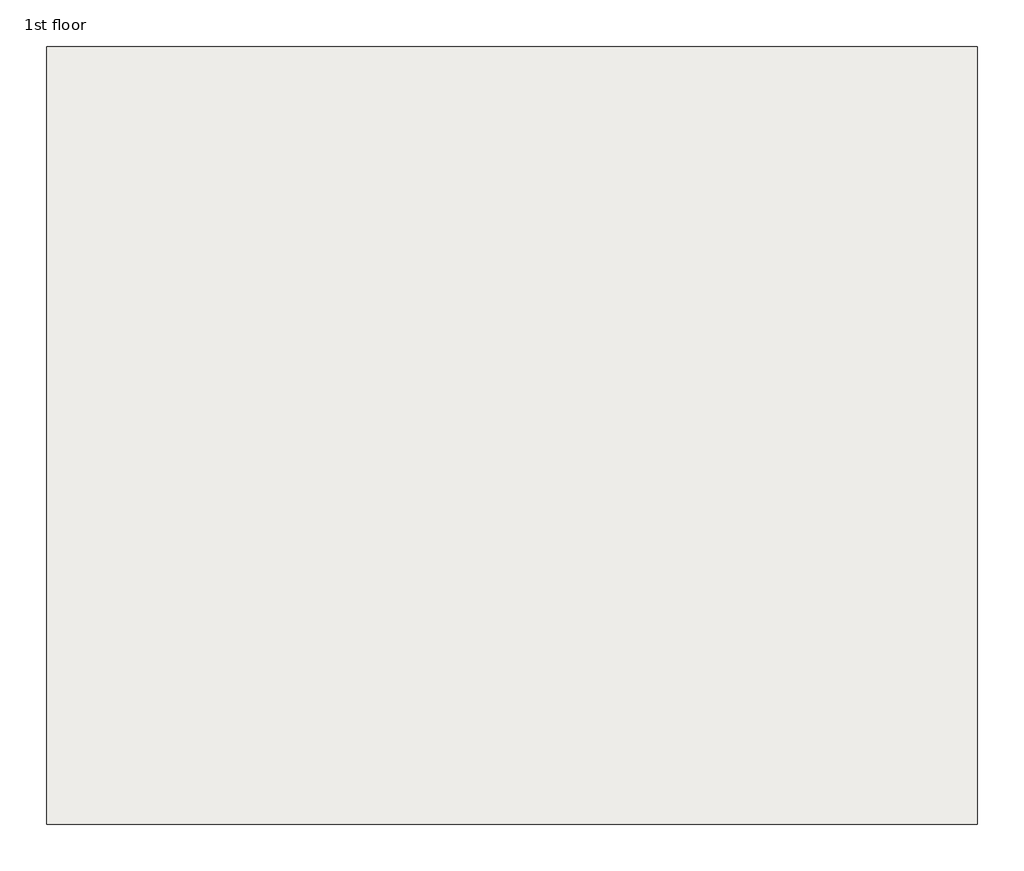
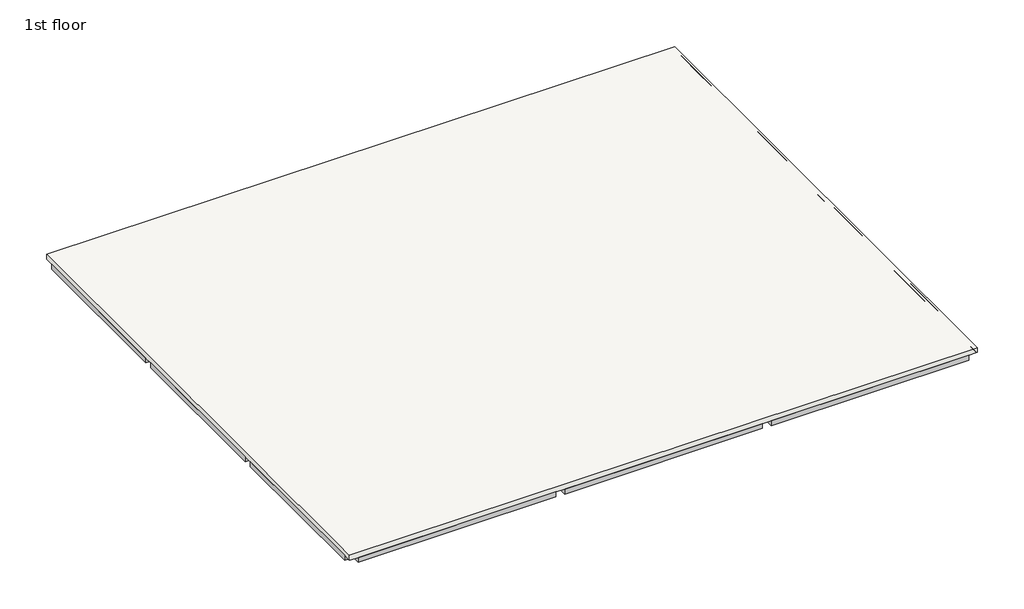
# One storey, part 1 of 2: 24 beams, 1 slab.
"""IFC4 building model written with IfcOpenShell, lengths in millimetres."""

from ifc_helpers import new_model, si_unit, frame, origin, place, context, project, spatial, polyline, outline, extrude, faceted_brep, element, save

model = new_model("IFC4")

# Units and contexts
model_context = context("Model", 3, world=origin())
ifc_project = project(units=[si_unit("LENGTHUNIT", "METRE", prefix="MILLI")], contexts=[model_context])

# Site, building, storey
site = spatial("IfcSite", under=ifc_project)
building = spatial("IfcBuilding", under=site)
storey = spatial("IfcBuildingStorey", under=building, Name="1st floor", Elevation=5000.0)

# Beams
placement = place(None, origin())
element("IfcBeam", 1, ObjectType="Concrete-Rectangular Beam : 250 x 300mm", at=placement, inside=storey, context=model_context, shape_type="SweptSolid", body=[
    extrude(outline(polyline([(-8833.7181639, -5693.2383613), (-8833.7181639, -5443.2383613), (-3083.7181639, -5443.2383613), (-3083.7181639, -5693.2383613), (-8833.7181639, -5693.2383613)])), frame((0.0, 0.0, 4700.0), z_axis=(0.0, 0.0, 1.0), x_axis=(1.0, 0.0, 0.0)), (0.0, 0.0, 1.0), 150.0),
])
element("IfcBeam", 2, ObjectType="Concrete-Rectangular Beam : 250 x 300mm", at=placement, inside=storey, context=model_context, shape_type="SweptSolid", body=[
    extrude(outline(polyline([(-2833.7181639, -5693.2383613), (-2833.7181639, -5443.2383613), (2916.2818361, -5443.2383613), (2916.2818361, -5693.2383613), (-2833.7181639, -5693.2383613)])), frame((0.0, 0.0, 4700.0), z_axis=(0.0, 0.0, 1.0), x_axis=(1.0, 0.0, 0.0)), (0.0, 0.0, 1.0), 150.0),
])
element("IfcBeam", 3, ObjectType="Concrete-Rectangular Beam : 250 x 300mm", at=placement, inside=storey, context=model_context, shape_type="SweptSolid", body=[
    extrude(outline(polyline([(3166.2818361, -5693.2383613), (3166.2818361, -5443.2383613), (8916.2818361, -5443.2383613), (8916.2818361, -5693.2383613), (3166.2818361, -5693.2383613)])), frame((0.0, 0.0, 4700.0), z_axis=(0.0, 0.0, 1.0), x_axis=(1.0, 0.0, 0.0)), (0.0, 0.0, 1.0), 150.0),
])
element("IfcBeam", 4, ObjectType="Concrete-Rectangular Beam : 250 x 300mm", at=placement, inside=storey, context=model_context, shape_type="SweptSolid", body=[
    extrude(outline(polyline([(-8833.7181639, -5693.2383613), (-8833.7181639, -10443.2383613), (-9083.7181639, -10443.2383613), (-9083.7181639, -5693.2383613), (-8833.7181639, -5693.2383613)])), frame((0.0, 0.0, 4700.0), z_axis=(0.0, 0.0, 1.0), x_axis=(1.0, 0.0, 0.0)), (0.0, 0.0, 1.0), 150.0),
])
element("IfcBeam", 5, ObjectType="Concrete-Rectangular Beam : 250 x 300mm", at=placement, inside=storey, context=model_context, shape_type="SweptSolid", body=[
    extrude(outline(polyline([(-8833.7181639, -10693.2383613), (-8833.7181639, -15443.2383613), (-9083.7181639, -15443.2383613), (-9083.7181639, -10693.2383613), (-8833.7181639, -10693.2383613)])), frame((0.0, 0.0, 4700.0), z_axis=(0.0, 0.0, 1.0), x_axis=(1.0, 0.0, 0.0)), (0.0, 0.0, 1.0), 150.0),
])
element("IfcBeam", 6, ObjectType="Concrete-Rectangular Beam : 250 x 300mm", at=placement, inside=storey, context=model_context, shape_type="SweptSolid", body=[
    extrude(outline(polyline([(-8833.7181639, -15693.2383613), (-8833.7181639, -20443.2383613), (-9083.7181639, -20443.2383613), (-9083.7181639, -15693.2383613), (-8833.7181639, -15693.2383613)])), frame((0.0, 0.0, 4700.0), z_axis=(0.0, 0.0, 1.0), x_axis=(1.0, 0.0, 0.0)), (0.0, 0.0, 1.0), 150.0),
])
element("IfcBeam", 7, ObjectType="Concrete-Rectangular Beam : 250 x 300mm", at=placement, inside=storey, context=model_context, shape_type="SweptSolid", body=[
    extrude(outline(polyline([(-3083.7181639, -10443.2383613), (-3083.7181639, -5693.2383613), (-2833.7181639, -5693.2383613), (-2833.7181639, -10443.2383613), (-3083.7181639, -10443.2383613)])), frame((0.0, 0.0, 4700.0), z_axis=(0.0, 0.0, 1.0), x_axis=(1.0, 0.0, 0.0)), (0.0, 0.0, 1.0), 150.0),
])
element("IfcBeam", 8, ObjectType="Concrete-Rectangular Beam : 250 x 300mm", at=placement, inside=storey, context=model_context, shape_type="SweptSolid", body=[
    extrude(outline(polyline([(-3083.7181639, -15443.2383613), (-3083.7181639, -10693.2383613), (-3058.7181639, -10693.2383613), (-3058.7181639, -15443.2383613), (-3083.7181639, -15443.2383613)])), frame((0.0, 0.0, 4700.0), z_axis=(0.0, 0.0, 1.0), x_axis=(1.0, 0.0, 0.0)), (0.0, 0.0, 1.0), 150.0),
    extrude(outline(polyline([(-2833.7181639, -10693.2383613), (-2833.7181639, -15443.2383613), (-2858.7181639, -15443.2383613), (-2858.7181639, -10693.2383613), (-2833.7181639, -10693.2383613)])), frame((0.0, 0.0, 4700.0), z_axis=(0.0, 0.0, 1.0), x_axis=(1.0, 0.0, 0.0)), (0.0, 0.0, 1.0), 150.0),
])
element("IfcBeam", 9, ObjectType="Concrete-Rectangular Beam : 250 x 300mm", at=placement, inside=storey, context=model_context, shape_type="SweptSolid", body=[
    extrude(outline(polyline([(-3083.7181639, -20443.2383613), (-3083.7181639, -15693.2383613), (-2833.7181639, -15693.2383613), (-2833.7181639, -20443.2383613), (-3083.7181639, -20443.2383613)])), frame((0.0, 0.0, 4700.0), z_axis=(0.0, 0.0, 1.0), x_axis=(1.0, 0.0, 0.0)), (0.0, 0.0, 1.0), 150.0),
])
element("IfcBeam", 10, ObjectType="Concrete-Rectangular Beam : 250 x 300mm", at=placement, inside=storey, context=model_context, shape_type="SweptSolid", body=[
    extrude(outline(polyline([(2916.2818361, -10443.2383613), (2916.2818361, -5693.2383613), (3166.2818361, -5693.2383613), (3166.2818361, -10443.2383613), (2916.2818361, -10443.2383613)])), frame((0.0, 0.0, 4700.0), z_axis=(0.0, 0.0, 1.0), x_axis=(1.0, 0.0, 0.0)), (0.0, 0.0, 1.0), 150.0),
])
element("IfcBeam", 11, ObjectType="Concrete-Rectangular Beam : 250 x 300mm", at=placement, inside=storey, context=model_context, shape_type="SweptSolid", body=[
    extrude(outline(polyline([(2916.2818361, -15443.2383613), (2916.2818361, -10693.2383613), (2941.2818361, -10693.2383613), (2941.2818361, -15443.2383613), (2916.2818361, -15443.2383613)])), frame((0.0, 0.0, 4700.0), z_axis=(0.0, 0.0, 1.0), x_axis=(1.0, 0.0, 0.0)), (0.0, 0.0, 1.0), 150.0),
    extrude(outline(polyline([(3166.2818361, -10693.2383613), (3166.2818361, -15443.2383613), (3141.2818361, -15443.2383613), (3141.2818361, -10693.2383613), (3166.2818361, -10693.2383613)])), frame((0.0, 0.0, 4700.0), z_axis=(0.0, 0.0, 1.0), x_axis=(1.0, 0.0, 0.0)), (0.0, 0.0, 1.0), 150.0),
])
element("IfcBeam", 12, ObjectType="Concrete-Rectangular Beam : 250 x 300mm", at=placement, inside=storey, context=model_context, shape_type="SweptSolid", body=[
    extrude(outline(polyline([(2916.2818361, -20443.2383613), (2916.2818361, -15693.2383613), (3166.2818361, -15693.2383613), (3166.2818361, -20443.2383613), (2916.2818361, -20443.2383613)])), frame((0.0, 0.0, 4700.0), z_axis=(0.0, 0.0, 1.0), x_axis=(1.0, 0.0, 0.0)), (0.0, 0.0, 1.0), 150.0),
])
element("IfcBeam", 13, ObjectType="Concrete-Rectangular Beam : 250 x 300mm", at=placement, inside=storey, context=model_context, shape_type="SweptSolid", body=[
    extrude(outline(polyline([(8916.2818361, -10443.2383613), (8916.2818361, -5693.2383613), (9166.2818361, -5693.2383613), (9166.2818361, -10443.2383613), (8916.2818361, -10443.2383613)])), frame((0.0, 0.0, 4700.0), z_axis=(0.0, 0.0, 1.0), x_axis=(1.0, 0.0, 0.0)), (0.0, 0.0, 1.0), 150.0),
])
element("IfcBeam", 14, ObjectType="Concrete-Rectangular Beam : 250 x 300mm", at=placement, inside=storey, context=model_context, shape_type="SweptSolid", body=[
    extrude(outline(polyline([(8916.2818361, -15443.2383613), (8916.2818361, -10693.2383613), (9166.2818361, -10693.2383613), (9166.2818361, -15443.2383613), (8916.2818361, -15443.2383613)])), frame((0.0, 0.0, 4700.0), z_axis=(0.0, 0.0, 1.0), x_axis=(1.0, 0.0, 0.0)), (0.0, 0.0, 1.0), 150.0),
])
element("IfcBeam", 15, ObjectType="Concrete-Rectangular Beam : 250 x 300mm", at=placement, inside=storey, context=model_context, shape_type="SweptSolid", body=[
    extrude(outline(polyline([(8916.2818361, -20443.2383613), (8916.2818361, -15693.2383613), (9166.2818361, -15693.2383613), (9166.2818361, -20443.2383613), (8916.2818361, -20443.2383613)])), frame((0.0, 0.0, 4700.0), z_axis=(0.0, 0.0, 1.0), x_axis=(1.0, 0.0, 0.0)), (0.0, 0.0, 1.0), 150.0),
])
element("IfcBeam", 16, ObjectType="Concrete-Rectangular Beam : 250 x 300mm", at=placement, inside=storey, context=model_context, shape_type="SweptSolid", body=[
    extrude(outline(polyline([(-8833.7181639, -20443.2383613), (-3083.7181639, -20443.2383613), (-3083.7181639, -20693.2383613), (-8833.7181639, -20693.2383613), (-8833.7181639, -20443.2383613)])), frame((0.0, 0.0, 4700.0), z_axis=(0.0, 0.0, 1.0), x_axis=(1.0, 0.0, 0.0)), (0.0, 0.0, 1.0), 150.0),
])
element("IfcBeam", 17, ObjectType="Concrete-Rectangular Beam : 250 x 300mm", at=placement, inside=storey, context=model_context, shape_type="SweptSolid", body=[
    extrude(outline(polyline([(-2833.7181639, -20443.2383613), (2916.2818361, -20443.2383613), (2916.2818361, -20693.2383613), (-2833.7181639, -20693.2383613), (-2833.7181639, -20443.2383613)])), frame((0.0, 0.0, 4700.0), z_axis=(0.0, 0.0, 1.0), x_axis=(1.0, 0.0, 0.0)), (0.0, 0.0, 1.0), 150.0),
])
element("IfcBeam", 18, ObjectType="Concrete-Rectangular Beam : 250 x 300mm", at=placement, inside=storey, context=model_context, shape_type="SweptSolid", body=[
    extrude(outline(polyline([(3166.2818361, -20443.2383613), (8916.2818361, -20443.2383613), (8916.2818361, -20693.2383613), (3166.2818361, -20693.2383613), (3166.2818361, -20443.2383613)])), frame((0.0, 0.0, 4700.0), z_axis=(0.0, 0.0, 1.0), x_axis=(1.0, 0.0, 0.0)), (0.0, 0.0, 1.0), 150.0),
])
element("IfcBeam", 19, ObjectType="Concrete-Rectangular Beam : 250 x 300mm", at=placement, inside=storey, context=model_context, shape_type="SweptSolid", body=[
    extrude(outline(polyline([(-8833.7181639, -15443.2383613), (-3083.7181639, -15443.2383613), (-3083.7181639, -15693.2383613), (-8833.7181639, -15693.2383613), (-8833.7181639, -15443.2383613)])), frame((0.0, 0.0, 4700.0), z_axis=(0.0, 0.0, 1.0), x_axis=(1.0, 0.0, 0.0)), (0.0, 0.0, 1.0), 150.0),
])
element("IfcBeam", 20, ObjectType="Concrete-Rectangular Beam : 250 x 300mm", at=placement, inside=storey, context=model_context, shape_type="SweptSolid", body=[
    extrude(outline(polyline([(2916.2818361, -15693.2383613), (-2833.7181639, -15693.2383613), (-2833.7181639, -15668.2383613), (2916.2818361, -15668.2383613), (2916.2818361, -15693.2383613)])), frame((0.0, 0.0, 4700.0), z_axis=(0.0, 0.0, 1.0), x_axis=(1.0, 0.0, 0.0)), (0.0, 0.0, 1.0), 150.0),
    extrude(outline(polyline([(-2833.7181639, -15443.2383613), (2916.2818361, -15443.2383613), (2916.2818361, -15468.2383613), (-2833.7181639, -15468.2383613), (-2833.7181639, -15443.2383613)])), frame((0.0, 0.0, 4700.0), z_axis=(0.0, 0.0, 1.0), x_axis=(1.0, 0.0, 0.0)), (0.0, 0.0, 1.0), 150.0),
])
element("IfcBeam", 21, ObjectType="Concrete-Rectangular Beam : 250 x 300mm", at=placement, inside=storey, context=model_context, shape_type="SweptSolid", body=[
    extrude(outline(polyline([(3166.2818361, -15693.2383613), (3166.2818361, -15443.2383613), (8916.2818361, -15443.2383613), (8916.2818361, -15693.2383613), (3166.2818361, -15693.2383613)])), frame((0.0, 0.0, 4700.0), z_axis=(0.0, 0.0, 1.0), x_axis=(1.0, 0.0, 0.0)), (0.0, 0.0, 1.0), 150.0),
])
element("IfcBeam", 22, ObjectType="Concrete-Rectangular Beam : 250 x 300mm", at=placement, inside=storey, context=model_context, shape_type="SweptSolid", body=[
    extrude(outline(polyline([(-8833.7181639, -10443.2383613), (-3083.7181639, -10443.2383613), (-3083.7181639, -10693.2383613), (-8833.7181639, -10693.2383613), (-8833.7181639, -10443.2383613)])), frame((0.0, 0.0, 4700.0), z_axis=(0.0, 0.0, 1.0), x_axis=(1.0, 0.0, 0.0)), (0.0, 0.0, 1.0), 150.0),
])
element("IfcBeam", 23, ObjectType="Concrete-Rectangular Beam : 250 x 300mm", at=placement, inside=storey, context=model_context, shape_type="SweptSolid", body=[
    extrude(outline(polyline([(2916.2818361, -10693.2383613), (-2833.7181639, -10693.2383613), (-2833.7181639, -10668.2383613), (2916.2818361, -10668.2383613), (2916.2818361, -10693.2383613)])), frame((0.0, 0.0, 4700.0), z_axis=(0.0, 0.0, 1.0), x_axis=(1.0, 0.0, 0.0)), (0.0, 0.0, 1.0), 150.0),
    extrude(outline(polyline([(-2833.7181639, -10443.2383613), (2916.2818361, -10443.2383613), (2916.2818361, -10468.2383613), (-2833.7181639, -10468.2383613), (-2833.7181639, -10443.2383613)])), frame((0.0, 0.0, 4700.0), z_axis=(0.0, 0.0, 1.0), x_axis=(1.0, 0.0, 0.0)), (0.0, 0.0, 1.0), 150.0),
])
element("IfcBeam", 24, ObjectType="Concrete-Rectangular Beam : 250 x 300mm", at=placement, inside=storey, context=model_context, shape_type="SweptSolid", body=[
    extrude(outline(polyline([(3166.2818361, -10693.2383613), (3166.2818361, -10443.2383613), (8916.2818361, -10443.2383613), (8916.2818361, -10693.2383613), (3166.2818361, -10693.2383613)])), frame((0.0, 0.0, 4700.0), z_axis=(0.0, 0.0, 1.0), x_axis=(1.0, 0.0, 0.0)), (0.0, 0.0, 1.0), 150.0),
])

# Slab
element("IfcSlab", 25, ObjectType="150mm Foundation Slab", at=placement, inside=storey, context=model_context, shape_type="Brep", body=[
    faceted_brep([(-9083.7181639, -5443.2383613, 4850.0), (-8833.7181639, -5443.2383613, 4850.0), (-3083.7181639, -5443.2383613, 4850.0), (-2833.7181639, -5443.2383613, 4850.0), (2916.2818361, -5443.2383613, 4850.0), (3166.2818361, -5443.2383613, 4850.0), (8916.2818361, -5443.2383613, 4850.0), (9166.2818361, -5443.2383613, 4850.0), (9166.2818361, -5693.2383613, 4850.0), (9166.2818361, -10443.2383613, 4850.0), (9166.2818361, -10693.2383613, 4850.0), (9166.2818361, -15443.2383613, 4850.0), (9166.2818361, -15693.2383613, 4850.0), (9166.2818361, -20443.2383613, 4850.0), (9166.2818361, -20693.2383613, 4850.0), (8916.2818361, -20693.2383613, 4850.0), (3166.2818361, -20693.2383613, 4850.0), (2916.2818361, -20693.2383613, 4850.0), (-2833.7181639, -20693.2383613, 4850.0), (-3083.7181639, -20693.2383613, 4850.0), (-8833.7181639, -20693.2383613, 4850.0), (-9083.7181639, -20693.2383613, 4850.0), (-9083.7181639, -20443.2383613, 4850.0), (-9083.7181639, -15693.2383613, 4850.0), (-9083.7181639, -15443.2383613, 4850.0), (-9083.7181639, -10693.2383613, 4850.0), (-9083.7181639, -10443.2383613, 4850.0), (-9083.7181639, -5693.2383613, 4850.0), (-9083.7181639, -5443.2383613, 5000.0), (-9083.7181639, -20693.2383613, 5000.0), (9166.2818361, -20693.2383613, 5000.0), (9166.2818361, -5443.2383613, 5000.0)], [[[0, 1, 2, 3, 4, 5, 6, 7, 8, 9, 10, 11, 12, 13, 14, 15, 16, 17, 18, 19, 20, 21, 22, 23, 24, 25, 26, 27]], [[28, 29, 30, 31]], [[7, 6, 5, 4, 3, 2, 1, 0, 28, 31]], [[14, 13, 12, 11, 10, 9, 8, 7, 31, 30]], [[21, 20, 19, 18, 17, 16, 15, 14, 30, 29]], [[0, 27, 26, 25, 24, 23, 22, 21, 29, 28]]]),
])

save(model, "model.ifc")

# Revit data of these elements
# Type "Concrete-Rectangular Beam : 250 x 300mm"
#   Length [instance default] = 1524 mm
#   b = 250 mm
#   h = 300 mm
#   Structural Material [instance default] = Concrete, Cast-in-Place gray
#   Assembly Code = ""
# Type "150mm Foundation Slab"
#   Layers, outside or top first: 150 mm "Concrete, Cast-in-Place gray" (function 1)
# Elements 1, 2, 3, 4, 5, 6, 7, 8, 9, 10, 11, 12, 13, 14, 15, 16, 17, 18, 19, 20, 21, 22, 23, 24 (IfcBeam, "Concrete-Rectangular Beam : 250 x 300mm")
#   Structural Material = Concrete, Cast-in-Place gray
#   Phase Created = New Construction
#   Materials on its faces: "Concrete, Cast-in-Place gray"
# Element 25 (IfcSlab, "150mm Foundation Slab")
#   built-in parameter 1001955 = 3.14159 (stored number, unit not read)
#   Height Offset From Level = 0 mm
#   built-in parameter 1001954 = 1
#   Phase Created = New Construction
#   Materials on its faces: "Concrete, Cast-in-Place gray"
# Materials
#   "Concrete, Cast-in-Place gray": class "Concrete", colour RGB 192 192 192, transparency 0, Description = "Cast-in-place concrete", Cost = 0
